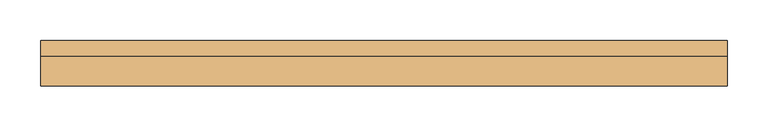
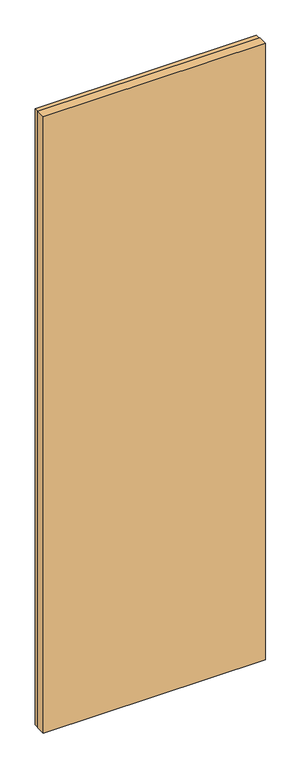
"""IFC4 building model written with IfcOpenShell, lengths in millimetres: door geometry, Anta Singola SENZA MANIGLIA(1) : Anta Singola SENZA MANIGLIA(1)."""

from ifc_helpers import new_model, si_unit, frame, origin, place, context, project, spatial, polyline, outline, extrude, source, transform, mapped, element, save


def door_af5377d0(model_context):
    return source(origin(), model_context, "Body", "SweptSolid", [
        extrude(outline(polyline([(422.5, 18.0), (422.5, -18.0), (-422.5, -18.0), (-422.5, 18.0), (422.5, 18.0)])), frame((0.0, 0.0, -3.1739529), z_axis=(0.0, 0.0, 1.0), x_axis=(1.0, 0.0, 0.0)), (0.0, 0.0, 1.0), 2478.1739529),
        extrude(outline(polyline([(2474.5625024, -422.0625024), (-2.7364552, -422.0625024), (-2.7364552, 422.0625024), (2474.5625024, 422.0625024), (2474.5625024, -422.0625024)]), holes=[polyline([(2429.5625024, 377.0625024), (42.2635448, 377.0625024), (42.2635448, -377.0625024), (2429.5625024, -377.0625024), (2429.5625024, 377.0625024)])]), frame((0.0, 18.0, 0.0), z_axis=(0.0, 1.0, 0.0), x_axis=(0.0, 0.0, 1.0)), (0.0, 0.0, 1.0), 20.0),
    ])


if __name__ == "__main__":
    model = new_model("IFC4")
    model_context = context("Model", 3, world=origin())
    ifc_project = project(units=[si_unit("LENGTHUNIT", "METRE", prefix="MILLI")], contexts=[model_context])
    site = spatial("IfcSite", under=ifc_project)
    building = spatial("IfcBuilding", under=site)
    placement = place(None, origin())
    door_shape = door_af5377d0(model_context)
    element("IfcDoor", 1, ObjectType="Anta Singola SENZA MANIGLIA(1) : Anta Singola SENZA MANIGLIA(1)", at=placement, inside=building, context=model_context, shape_type="MappedRepresentation", body=[
        mapped(door_shape, transform((0.0, 0.0, 0.0), x_axis=(1.0, 0.0, 0.0), y_axis=(0.0, 1.0, 0.0), z_axis=(0.0, 0.0, 1.0))),
    ])
    save(model, "model.ifc")

# Revit data of these elements
# Type "Anta Singola SENZA MANIGLIA(1) : Anta Singola SENZA MANIGLIA(1)"
#   Type Mark = "15"
#   Construction Type = "Scorrimenti"
#   Construction Type Id = "opn-d42"
#   Analytic Construction = "Telaio in metallo con vetro singolo trasparente"
#   Sp = 0.036 m
#   Thermal Resistance (R) = 0.152486 (m²·K)/W
#   Heat Transfer Coefficient (U) = 6.5580 W/(m²·K)
#   L cornice = 0.045 m
#   Quadro = Default - Vetro
#   Maniglia = none
#   Visual Light Transmittance = 0
#   Solar Heat Gain Coefficient = 0
#   Manufacturer = ""
#   Function = (empty or 0)
# Element 1 (IfcDoor, "Anta Singola SENZA MANIGLIA(1) : Anta Singola SENZA MANIGLIA(1)")
#   Materials on its faces: "Maniglia", "Default - Vetro"
# Materials
#   "Default - Vetro": class "Vetro", colour RGB 208 208 208, transparency 0.7, Cost = 0
#   "Maniglia": class "Varie", colour RGB 219 219 219, transparency 0
